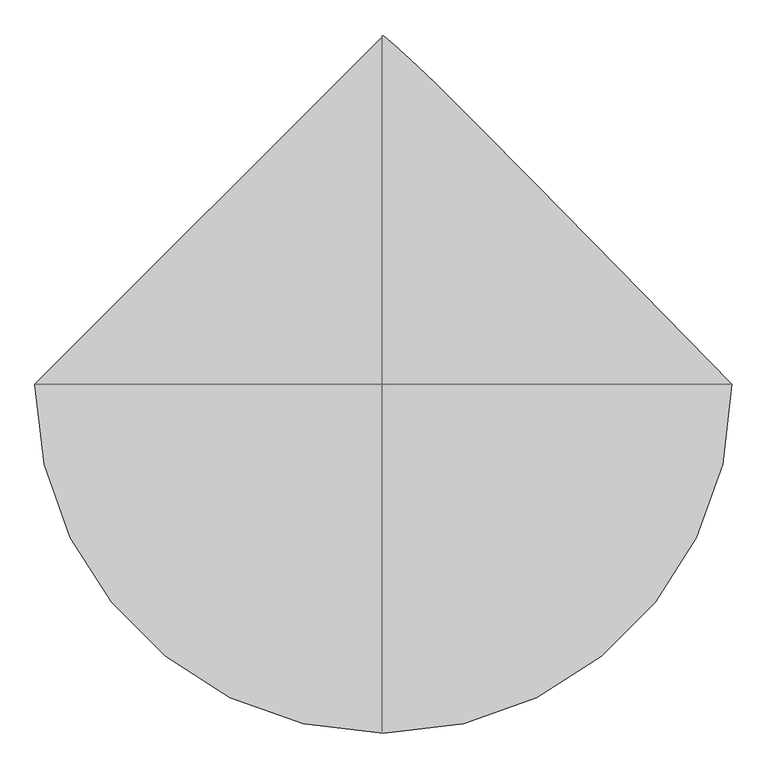
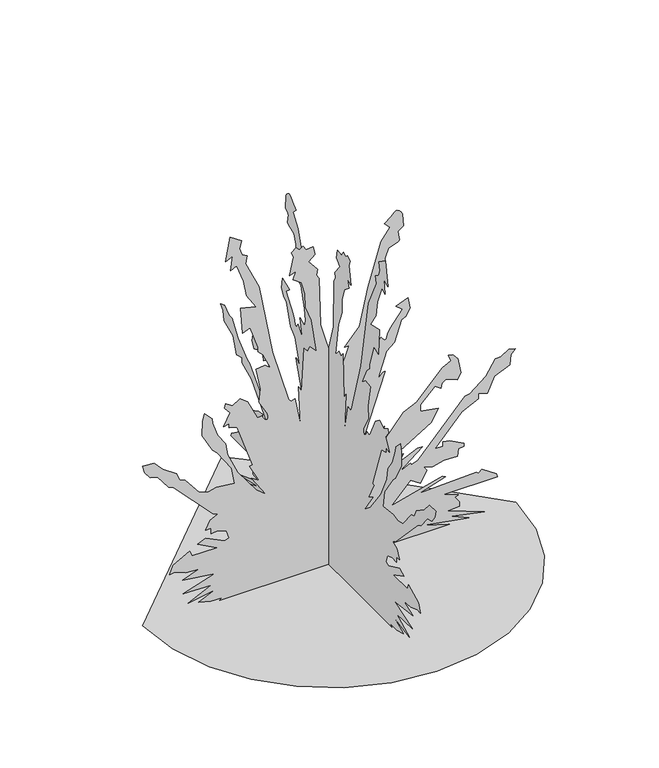
"""IFC4 building model written with IfcOpenShell, lengths in millimetres: proxy geometry, maiden grass 26738 : maiden grass 26738."""

import ifcopenshell
import ifcopenshell.guid

model = None  # the IFC model being written
_history = None  # IfcOwnerHistory: only IFC2X3 demands one
_inside = {}  # id of a spatial element -> (the spatial element, [elements in it])
_under = {}  # id of a project, library or spatial element -> (it, [spatial elements below it])
_declared = {}  # id of a project -> (the project, [libraries it declares])
_typed = {}  # id of a type object -> (the type object, [elements of that type])
_made_of = {}  # id of a material, layer set ... -> (it, [elements and type objects made of it])


def new_model(schema):
    """Start an empty IFC model of exactly this schema.

    Asked for "IFC4X3", IfcOpenShell would pick the latest addendum, in which some entities
    have other attributes; the version numbers below select the first issue.
    IFC2X3 requires an IfcOwnerHistory on every rooted entity: one is made here for all.
    """
    global model, _history
    if schema == "IFC4X3":
        model = ifcopenshell.file(schema_version=(4, 3, 0, 0))
    else:
        model = ifcopenshell.file(schema=schema)
    _inside.clear()
    _under.clear()
    _declared.clear()
    _typed.clear()
    _made_of.clear()
    _history = None
    if model.schema == "IFC2X3":
        org = make("IfcOrganization", Name="unknown")
        user = make(
            "IfcPersonAndOrganization",
            ThePerson=make("IfcPerson", FamilyName="unknown"),
            TheOrganization=org,
        )
        app = make(
            "IfcApplication",
            ApplicationDeveloper=org,
            Version="unknown",
            ApplicationFullName="unknown",
            ApplicationIdentifier="unknown",
        )
        _history = make(
            "IfcOwnerHistory",
            OwningUser=user,
            OwningApplication=app,
            ChangeAction="ADDED",
            CreationDate=0,
        )
    return model


def make(cls, **values):
    """One entity of the class cls with the attributes given. An attribute that is None is left unset."""
    return model.create_entity(
        cls, **{name: value for name, value in values.items() if value is not None}
    )


def rooted(cls, **values):
    """An entity with a GlobalId (a new one), such as an element, a storey or a relation."""
    return make(cls, GlobalId=ifcopenshell.guid.new(), OwnerHistory=_history, **values)


def si_unit(unit_type, name, prefix=None):
    """IfcSIUnit, for example si_unit("LENGTHUNIT", "METRE", prefix="MILLI")."""
    return make("IfcSIUnit", UnitType=unit_type, Prefix=prefix, Name=name)


def assignment(units):
    """IfcUnitAssignment: the units of a project."""
    return None if units is None else make("IfcUnitAssignment", Units=units)


def point(xyz):
    """IfcCartesianPoint."""
    return None if xyz is None else make("IfcCartesianPoint", Coordinates=xyz)


def direction(xyz):
    """IfcDirection."""
    return None if xyz is None else make("IfcDirection", DirectionRatios=xyz)


def frame(location, z_axis=None, x_axis=None):
    """IfcAxis2Placement3D, a coordinate frame: its origin and axes. An axis left out is left unset."""
    return make(
        "IfcAxis2Placement3D",
        Location=point(location),
        Axis=direction(z_axis),
        RefDirection=direction(x_axis),
    )


def origin():
    """The frame at (0, 0, 0) with its axes left unset."""
    return frame((0.0, 0.0, 0.0))


def place(relative_to, where):
    """IfcLocalPlacement: puts the frame where relative to a parent placement (None: the world)."""
    return make(
        "IfcLocalPlacement", PlacementRelTo=relative_to, RelativePlacement=where
    )


def context(
    kind, dimensions, precision=None, world=None, true_north=None, identifier=None
):
    """IfcGeometricRepresentationContext, for example the 3D "Model" context."""
    return make(
        "IfcGeometricRepresentationContext",
        ContextIdentifier=identifier,
        ContextType=kind,
        CoordinateSpaceDimension=dimensions,
        Precision=precision,
        WorldCoordinateSystem=world,
        TrueNorth=true_north,
    )


def project(units=None, contexts=None):
    """IfcProject with its units and contexts."""
    return rooted(
        "IfcProject",
        Name="project",
        RepresentationContexts=contexts,
        UnitsInContext=assignment(units),
    )


def spatial(cls, under=None, at=None, **own):
    """A site, building, storey or space (cls), placed at a placement, below another one or the project."""
    s = rooted(cls, ObjectPlacement=at, **own)
    if under is not None:
        _under.setdefault(under.id(), (under, []))[1].append(s)
    return s


def point_list(points):
    """IfcCartesianPointList2D or 3D."""
    cls = (
        "IfcCartesianPointList2D" if len(points[0]) == 2 else "IfcCartesianPointList3D"
    )
    return make(cls, CoordList=points)


def triangles(points, corners, closed=None, point_numbers=None):
    """IfcTriangulatedFaceSet: each triangle names its three corners, points numbered from 1."""
    return make(
        "IfcTriangulatedFaceSet",
        Coordinates=point_list(points),
        Closed=closed,
        CoordIndex=corners,
        PnIndex=point_numbers,
    )


def shape(context_of_items, identifier, shape_type, items):
    """IfcShapeRepresentation: the items that make up one representation, for example the "Body"."""
    return make(
        "IfcShapeRepresentation",
        ContextOfItems=context_of_items,
        RepresentationIdentifier=identifier,
        RepresentationType=shape_type,
        Items=items,
    )


def source(mapping_origin, context_of_items, identifier, shape_type, items):
    """IfcRepresentationMap: a shape defined once, which mapped items show again and again."""
    return make(
        "IfcRepresentationMap",
        MappingOrigin=mapping_origin,
        MappedRepresentation=shape(context_of_items, identifier, shape_type, items),
    )


def transform(
    local_origin,
    x_axis=None,
    y_axis=None,
    z_axis=None,
    scale=None,
    scale2=None,
    scale3=None,
    uniform=True,
):
    """IfcCartesianTransformationOperator3D, or its non-uniform kind. x_axis, y_axis, z_axis: its Axis1, 2, 3."""
    if uniform:
        return make(
            "IfcCartesianTransformationOperator3D",
            Axis1=direction(x_axis),
            Axis2=direction(y_axis),
            LocalOrigin=point(local_origin),
            Scale=scale,
            Axis3=direction(z_axis),
        )
    return make(
        "IfcCartesianTransformationOperator3DnonUniform",
        Axis1=direction(x_axis),
        Axis2=direction(y_axis),
        LocalOrigin=point(local_origin),
        Scale=scale,
        Axis3=direction(z_axis),
        Scale2=scale2,
        Scale3=scale3,
    )


def mapped(mapping_source, mapping_target):
    """IfcMappedItem: shows the shape of a source again, moved by a transform."""
    return make(
        "IfcMappedItem", MappingSource=mapping_source, MappingTarget=mapping_target
    )


def made_of(thing, what):
    """Note that an element or type object is made of a material, layer set ...; save() writes the relation."""
    if what is not None:
        _made_of.setdefault(what.id(), (what, []))[1].append(thing)
    return thing


def element(
    cls,
    number,
    at=None,
    inside=None,
    cuts=None,
    type_object=None,
    material=None,
    context=None,
    identifier="Body",
    shape_type=None,
    held_by="IfcProductDefinitionShape",
    body=None,
    shapes=None,
    **own,
):
    """One element of the class cls, such as IfcWall. Its Tag is "e" and its number.

    at: its placement. inside: the storey or other place that contains it. cuts: it is an
    opening in that element (IfcRelVoidsElement). A single representation is given by context,
    identifier, shape_type and body (its items); several are given by shapes. held_by: the class
    of the entity that holds the representations. save() writes the other relations.
    """
    e = rooted(cls, Tag="e%d" % number, ObjectPlacement=at, **own)
    if body is not None:
        shapes = [shape(context, identifier, shape_type, body)]
    if shapes is not None:
        e.Representation = make(held_by, Representations=shapes)
    if inside is not None:
        _inside.setdefault(inside.id(), (inside, []))[1].append(e)
    if cuts is not None:
        rooted(
            "IfcRelVoidsElement", RelatingBuildingElement=cuts, RelatedOpeningElement=e
        )
    if type_object is not None:
        _typed.setdefault(type_object.id(), (type_object, []))[1].append(e)
    return made_of(e, material)


def aggregate(whole, parts):
    """IfcRelAggregates: a whole, such as a stair, and the parts it consists of."""
    return rooted("IfcRelAggregates", RelatingObject=whole, RelatedObjects=parts)


def save(model, path):
    """Write the relations noted so far, then the file.

    IfcRelAggregates (storeys below a building ...), IfcRelContainedInSpatialStructure (elements
    in a storey), IfcRelDefinesByType, IfcRelAssociatesMaterial and IfcRelDeclares: one each for
    every whole, place, type object, material and project.
    """
    for whole, parts in _under.values():
        aggregate(whole, parts)
    for where, things in _inside.values():
        rooted(
            "IfcRelContainedInSpatialStructure",
            RelatedElements=things,
            RelatingStructure=where,
        )
    for kind, things in _typed.values():
        rooted("IfcRelDefinesByType", RelatedObjects=things, RelatingType=kind)
    for what, things in _made_of.values():
        rooted("IfcRelAssociatesMaterial", RelatedObjects=things, RelatingMaterial=what)
    for by, libraries in _declared.values():
        rooted("IfcRelDeclares", RelatingContext=by, RelatedDefinitions=libraries)
    model.write(path)


def entourage_51d93d44(model_context):
    return source(origin(), model_context, "Body", "Tessellation", [
        triangles([(-822.1126825, 0.0, 0.0001374), (-800.3786167, -188.373858, 0.0001374), (-738.480578, -361.3651156, 0.0001374), (-641.3745867, -514.0173532, 0.0001374), (-514.0174622, -641.374732, 0.0001374), (-361.365043, -738.4805054, 0.0001374), (-188.3737671, -800.378544, 0.0001374), (3.59e-05, -822.1126825, 0.0001374), (188.3739125, -800.3786167, 0.0001374), (361.3651883, -738.480578, 0.0001374), (514.0174622, -641.3745867, 0.0001374), (641.3748047, -514.0174622, 0.0001374), (738.4805054, -361.365043, 0.0001374), (800.378544, -188.373749, 0.0001374), (822.1126825, 7.19e-05, 0.0001374), (554.9441065, 274.0493697, 0.0001374), (356.8788342, 475.8195757, 0.0001374), (216.3996546, 617.3571573, 0.0001374), (121.9894107, 710.7087994, 0.0001374), (62.1308551, 767.9210049, 0.0001374), (25.3067606, 801.0401316, 0.0001374), (-0.0001078, 822.1126825, 0.0001374), (-486.0236403, 7.81e-05, 0.9155915), (-471.7920599, 7.76e-05, 9.8343198), (-523.9165309, 7.76e-05, 9.7573804), (-575.3383922, 7.67e-05, 24.6529329), (-504.1805263, 7.48e-05, 56.6647099), (-622.6670803, 7.61e-05, 35.566252), (-521.099806, 7.32e-05, 83.8197293), (-644.3685173, 7.29e-05, 88.7502968), (-506.307395, 7.03e-05, 133.1254316), (-645.8895727, 6.92e-05, 151.363835), (-575.3383922, 6.76e-05, 177.5005391), (-633.4720894, 6.73e-05, 182.811861), (-682.2468012, 6.62e-05, 200.8128698), (-703.5376528, 6.64e-05, 197.2227365), (-688.7453144, 6.41e-05, 236.667331), (-614.7840586, 6.17e-05, 276.1118528), (-604.9224512, 6.32e-05, 251.4590335), (-494.8790591, 6.34e-05, 248.9685605), (-580.2687962, 6.06e-05, 295.8341047), (-545.7534247, 5.97e-05, 310.6258072), (-461.9305979, 6.2e-05, 271.1812672), (-442.4802589, 6.16e-05, 277.8612192), (-452.1878423, 5.96e-05, 312.2414789), (-492.5862848, 5.87e-05, 327.4185685), (-520.7920123, 5.89e-05, 323.5701842), (-521.099806, 5.73e-05, 350.0703109), (-545.7534247, 5.73e-05, 350.0703109), (-526.0308277, 5.5e-05, 389.5148872), (-491.515202, 5.41e-05, 404.3065716), (-513.2632931, 5.35e-05, 414.7085166), (-685.7770363, 4.26e-05, 596.5231456), (-707.8857159, 4.2e-05, 606.6573017), (-757.7759846, 3.82e-05, 670.5571804), (-790.6316099, 3.78e-05, 677.9690826), (-814.6804327, 3.58e-05, 711.7275599), (-821.8761417, 3.38e-05, 744.5156021), (-771.5802292, 3.4e-05, 740.8769434), (-734.9066683, 3.66e-05, 698.0076851), (-673.9536301, 3.91e-05, 655.7654961), (-659.1609283, 4.12e-05, 621.2515417), (-636.2393623, 4.16e-05, 613.9256081), (-573.062332, 4.63e-05, 535.429927), (-531.2541281, 4.7e-05, 522.9600486), (-496.445933, 4.65e-05, 532.501254), (-417.5538008, 4.7e-05, 522.6401553), (-431.8794525, 4.26e-05, 597.7539207), (-494.1621334, 3.7e-05, 691.4321417), (-515.1618327, 3.58e-05, 710.6897598), (-560.6032451, 3.08e-05, 794.7286709), (-559.6332461, 2.68e-05, 861.8978268), (-550.6847371, 2.5e-05, 892.4327362), (-516.1688933, 2.71e-05, 857.9187092), (-514.4276842, 2.84e-05, 836.1371899), (-492.5786181, 3.21e-05, 773.1969183), (-456.9999032, 3.53e-05, 719.8628918), (-448.1073864, 3.85e-05, 666.0661755), (-403.8973306, 4.42e-05, 569.7717261), (-322.5198123, 5.08e-05, 459.5990905), (-279.4932235, 5.29e-05, 424.0288053), (-341.7963246, 4.73e-05, 518.5882951), (-309.0772825, 4.85e-05, 497.987336), (-351.6489936, 4.37e-05, 579.3482491), (-338.6617049, 4.35e-05, 581.8069654), (-407.6923751, 3.18e-05, 779.0296291), (-442.2077102, 3.12e-05, 788.8907278), (-442.2077102, 3e-05, 808.6129978), (-466.8613289, 3.03e-05, 803.6824848), (-437.2769065, 2.71e-05, 857.9187092), (-461.9305979, 2.53e-05, 887.5020779), (-456.9999032, 2.41e-05, 907.2244205), (-427.4157715, 2.53e-05, 887.5020779), (-392.9001457, 2.41e-05, 907.2244205), (-361.3909862, 2.55e-05, 883.444622), (-319.5289701, 3.13e-05, 794.863619), (-316.5251201, 3.15e-05, 792.847681), (-312.9193082, 3.15e-05, 792.290593), (-308.9018935, 3.15e-05, 792.6843916), (-304.6633259, 3.13e-05, 793.5212591), (-300.3935829, 3.11e-05, 794.293523), (-296.2831507, 3.08e-05, 794.4932928), (-293.8821344, 3.1e-05, 789.7024515), (-291.6524922, 3.11e-05, 784.6016001), (-289.2939152, 3.13e-05, 779.6455799), (-286.5060222, 3.14e-05, 775.2894505), (-282.9887042, 3.16e-05, 771.9882711), (-278.4414163, 3.19e-05, 770.1969561), (-272.5639226, 3.23e-05, 770.3705647), (-270.4821274, 3.19e-05, 776.4802935), (-269.746798, 3.16e-05, 782.5422054), (-271.4178988, 3.09e-05, 794.5538269), (-309.0772825, 2.68e-05, 862.8492222), (-304.1468967, 2.32e-05, 922.0159595), (-323.8695119, 1.74e-05, 1020.6273823), (-284.423464, 1.71e-05, 1025.5578953), (-259.7697544, 1.82e-05, 1005.8357706), (-292.5143764, 1.4e-05, 1076.7667608), (-314.0080499, 1.27e-05, 1099.5164623), (-315.0547156, 1.15e-05, 1119.0795851), (-348.5233486, 5.3e-06, 1222.7807407), (-383.038502, 6.2e-06, 1207.9888384), (-391.1781941, -1e-06, 1327.8346481), (-323.8695119, 0.0, 1311.5309921), (-365.2547038, -3.9e-06, 1377.9884182), (-377.5616561, -8.2e-06, 1449.0455635), (-409.7759325, -1.31e-05, 1532.0531422), (-435.1933854, -1.24e-05, 1519.3450516), (-427.4157715, -1.61e-05, 1582.7118233), (-456.9999032, -1.53e-05, 1567.9204296), (-438.6445556, -2.17e-05, 1676.3998547), (-387.9694147, -1.97e-05, 1641.8788513), (-396.0815286, -1.75e-05, 1605.9381672), (-384.2218237, -1.56e-05, 1574.3406773), (-363.3155416, -1.5e-05, 1562.9896259), (-368.246309, -1.29e-05, 1528.4758896), (-309.0772825, -5.3e-06, 1400.2812435), (-250.6196225, 1.42e-05, 1073.5192846), (-180.2010283, 2.87e-05, 830.6251717), (-169.6161911, 2.95e-05, 817.4087545), (-151.2930636, 2.91e-05, 823.4046822), (-126.6192335, 3.68e-05, 694.4196774), (-136.5008433, 2.62e-05, 872.7103935), (-121.7086412, 2.76e-05, 848.0576105), (-111.8470156, 1.59e-05, 1045.2803106), (-97.0548044, 1.71e-05, 1025.5578953), (-84.6295182, 1.62e-05, 1040.6290684), (-57.6092516, 1.79e-05, 1010.7662109), (-79.5582798, 8.8e-06, 1163.7574539), (-104.4511553, 4.7e-06, 1232.6419121), (-107.5404289, 9e-07, 1296.0368797), (-123.4986664, -2.4e-06, 1352.177639), (-161.1545347, -4.1e-06, 1380.5586102), (-146.3623326, -6.2e-06, 1415.0727825), (-175.9469094, -5.6e-06, 1405.2116112), (-158.7234512, -1.03e-05, 1484.8167812), (-166.0854474, -1.17e-05, 1508.7534016), (-146.3623326, -1.26e-05, 1523.5452312), (-131.5704484, -1.17e-05, 1508.7534016), (-116.6065998, -1.25e-05, 1521.4754448), (-101.9855355, -1.11e-05, 1498.8923756), (-72.4009586, -1.14e-05, 1503.8230339), (-62.5394784, -9.1e-06, 1464.3783485), (-92.1240644, -7.6e-06, 1439.7256382), (-52.6780073, -4.7e-06, 1390.4200722), (-57.6092516, -3.2e-06, 1365.7670712), (-44.9584885, -2.1e-06, 1346.546006), (-40.1288097, 1.1e-05, 1128.143712), (16.3521246, 2.24e-05, 936.8077166), (25.6302442, 2.16e-05, 950.3199005), (46.3616142, 2.59e-05, 877.5758669), (85.383115, 1.94e-05, 986.1135006), (65.6596505, 1.94e-05, 986.1135006), (132.852038, 1.49e-05, 1062.0039265), (169.7376772, 4.9e-06, 1229.8971668), (228.245861, -6.6e-06, 1421.9566647), (267.8211162, -9.7e-06, 1474.2395199), (243.1672431, -1.11e-05, 1498.8923756), (272.0833378, -1.25e-05, 1521.3225471), (286.4673436, -1.31e-05, 1537.556876), (293.7374485, -1.35e-05, 1542.3155972), (297.4055931, -1.38e-05, 1543.2675739), (308.1376596, -1.27e-05, 1537.579549), (315.8437663, -1.16e-05, 1529.0826839), (321.0283699, -1.07e-05, 1518.2452641), (326.6370392, -7.7e-06, 1460.8509476), (306.7311321, -7.7e-06, 1447.4507481), (304.3311514, -7.7e-06, 1444.519241), (302.7936726, -7.7e-06, 1441.4505329), (309.1859605, -6.2e-06, 1402.4600349), (307.1584316, -5.9e-06, 1398.4450184), (302.9130694, -5.6e-06, 1394.7411747), (261.356885, -4e-06, 1379.0709103), (246.0123274, -1.6e-06, 1337.9506004), (244.0019305, 9e-07, 1296.3149151), (228.3094291, 3.3e-06, 1256.0202816), (220.8882069, 7.9e-06, 1179.9705631), (207.4437332, 6.8e-06, 1171.8723656), (179.3911032, 1.38e-05, 1079.9680189), (173.3980279, 1.7e-05, 1026.8490955), (180.4457445, 1.86e-05, 999.5491631), (213.582312, 1.77e-05, 1015.6967239), (193.859715, 2.26e-05, 931.8771309), (228.3750501, 2e-05, 976.2522566), (242.287573, 2.11e-05, 957.5074705), (251.845438, 2.09e-05, 961.1874784), (256.8526723, 1.97e-05, 980.8979033), (266.7142615, 1.85e-05, 1002.0413801), (322.059448, 1.41e-05, 1074.863534), (293.6769507, 1.28e-05, 1097.3908653), (346.713212, 1.15e-05, 1119.2386597), (354.6484835, 1.44e-05, 1069.6418324), (338.174271, 1.65e-05, 1035.8738354), (317.1287169, 1.71e-05, 1025.5578953), (287.5436224, 2.26e-05, 931.8771309), (252.1265254, 2.44e-05, 903.2333851), (213.582312, 3.12e-05, 788.8907278), (236.8349806, 3.03e-05, 809.7009401), (240.9621815, 3e-05, 811.6948591), (244.803971, 2.97e-05, 812.5061468), (244.8585279, 3e-05, 809.5433916), (134.690634, 4.91e-05, 488.1261283), (242.8606121, 4.5e-05, 557.2269977), (237.4122891, 4.6e-05, 540.8212403), (140.9250282, 5.13e-05, 450.6353934), (129.759903, 5.23e-05, 433.8900129), (164.2748021, 5.06e-05, 463.4733816), (174.1367001, 5.06e-05, 463.4733816), (159.0154937, 5.29e-05, 425.0493098), (238.8042827, 4.92e-05, 486.724506), (326.990179, 4.29e-05, 591.668064), (382.9130736, 4.13e-05, 618.7366516), (499.039125, 3.41e-05, 739.7414022), (534.9049227, 3.29e-05, 759.6449112), (524.2203278, 3.12e-05, 788.8907278), (544.510332, 3.15e-05, 783.3986212), (566.5761726, 3.31e-05, 756.7437075), (580.5672881, 3.72e-05, 688.0601091), (563.6663939, 3.88e-05, 660.6960091), (514.5438108, 3.76e-05, 681.3525244), (496.7209162, 3.83e-05, 668.9436161), (492.0994686, 3.96e-05, 646.9967726), (465.0513376, 3.85e-05, 665.6265947), (400.9515075, 4.23e-05, 601.5291627), (400.9515075, 4.41e-05, 571.9458303), (479.8436033, 4.5e-05, 557.154146), (450.2590719, 4.82e-05, 502.9179216), (287.5436224, 5.41e-05, 404.3065716), (325.8399585, 5.44e-05, 399.649116), (302.3363241, 5.64e-05, 364.8620679), (387.4521134, 5.41e-05, 404.7523293), (411.1211992, 5.41e-05, 403.6902938), (307.2671459, 5.91e-05, 320.4869785), (356.5747104, 5.76e-05, 345.1397979), (361.5048964, 5.82e-05, 335.2785539), (389.4130039, 5.74e-05, 348.2994524), (598.1816563, 4.41e-05, 571.9458303), (618.663909, 4.38e-05, 576.9850576), (688.6817282, 4.05e-05, 633.1896212), (731.3115389, 3.65e-05, 700.1405491), (755.9652666, 3.65e-05, 700.1405491), (790.4811104, 3.5e-05, 724.7934048), (820.0657145, 3.56e-05, 714.9323061), (800.3426451, 3.68e-05, 695.2100361), (795.4119141, 3.94e-05, 650.8349104), (726.3813166, 4.12e-05, 621.2515417), (696.7968578, 4.53e-05, 552.2235603), (657.3502831, 4.47e-05, 562.084659), (657.4310921, 4.61e-05, 538.9833801), (583.1111009, 4.8e-05, 506.1758986), (465.0513376, 5.59e-05, 374.7231666), (499.5666, 5.59e-05, 374.7231666), (499.5666, 5.47e-05, 394.4454366), (528.894134, 5.5e-05, 389.8867032), (593.2509616, 5.7e-05, 355.0009329), (593.2509616, 5.79e-05, 340.2092485), (568.4129791, 5.81e-05, 337.6585321), (563.6663939, 6e-05, 305.6952579), (504.8713271, 5.99e-05, 306.2484581), (453.6921109, 6.06e-05, 295.5878443), (415.7437732, 6e-05, 305.6952579), (430.5360752, 6.11e-05, 285.9729515), (400.9515075, 6.41e-05, 236.667331), (356.5747104, 6.23e-05, 266.2507178), (272.7518472, 6.76e-05, 177.5005391), (498.0560818, 6.42e-05, 234.1173413), (512.2016573, 6.46e-05, 227.2681409), (396.0207401, 6.67e-05, 192.2922235), (647.8657602, 6.62e-05, 201.1622852), (657.3502831, 6.67e-05, 192.2922235), (672.1430574, 6.59e-05, 207.083926), (736.2428513, 6.85e-05, 162.7088003), (741.1735823, 6.94e-05, 147.9171159), (499.5666, 6.94e-05, 147.9171159), (568.5971612, 7.08e-05, 123.2642602), (552.2703235, 7.12e-05, 117.9041314), (573.5278922, 7.29e-05, 88.7502968), (573.5278922, 7.41e-05, 69.0280223), (521.428892, 7.43e-05, 64.9850141), (682.0040108, 7.79e-05, 4.9306691), (539.0127025, 7.61e-05, 34.5140656), (617.9047256, 7.82e-05, 0.0001036), (415.7437732, 7.61e-05, 34.5140656), (529.1511314, 7.82e-05, 0.0001036), (-3.5682026, -482.4553988, 0.9154881), (-3.5682026, -468.2238184, 9.8342176), (-3.5682026, -520.3482894, 9.7572771), (-3.5682026, -571.770187, 24.652833), (-3.5682026, -500.6122484, 56.6646145), (-3.5682026, -619.0989115, 35.5661476), (-3.5682026, -517.5314919, 83.8196294), (-3.5682026, -640.8002758, 88.750206), (-3.5682026, -502.7391898, 133.1253407), (-3.5682026, -642.3213312, 151.3637533), (-3.5682026, -571.770187, 177.5004483), (-3.5682026, -629.9037752, 182.8117702), (-3.5682026, -678.6785597, 200.8127971), (-3.5682026, -699.9694839, 197.2226638), (-3.5682026, -685.1770729, 236.6672583), (-3.5682026, -611.2158897, 276.1117802), (-3.5682026, -601.3542097, 251.4589427), (-3.5682026, -491.310854, 248.9684878), (-3.5682026, -576.7005547, 295.8340138), (-3.5682026, -542.1852559, 310.6257345), (-3.5682026, -458.3623564, 271.1812308), (-3.5682026, -438.9119811, 277.8611647), (-3.5682026, -448.6196008, 312.2414426), (-3.5682026, -489.0179707, 327.4185322), (-3.5682026, -517.2238071, 323.5701479), (-3.5682026, -517.5314919, 350.0702745), (-3.5682026, -542.1852559, 350.0702745), (-3.5682026, -522.4626225, 389.5148509), (-3.5682026, -487.9469604, 404.3065352), (-3.5682026, -509.6950516, 414.7084803), (-3.5682026, -682.2087948, 596.5231456), (-3.5682026, -704.3174744, 606.6573017), (-3.5682026, -754.2077431, 670.5571804), (-3.5682026, -787.0633684, 677.9690826), (-3.5682026, -811.1121912, 711.7275599), (-3.5682026, -818.3079729, 744.5156021), (-3.5682026, -768.0119877, 740.8769434), (-3.5682026, -731.3384995, 698.0076851), (-3.5682026, -670.3853886, 655.7654961), (-3.5682026, -655.5926868, 621.251469), (-3.5682026, -632.6711208, 613.9256081), (-3.5682026, -569.4940905, 535.4298543), (-3.5682026, -527.6859229, 522.9599759), (-3.5682026, -492.8777278, 532.501254), (-3.5682026, -413.9855593, 522.6401553), (-3.5682026, -428.311211, 597.7538844), (-3.5682026, -490.5938556, 691.4321417), (-3.5682026, -511.5936275, 710.6897598), (-3.5682026, -557.0350036, 794.7286709), (-3.5682026, -556.0649683, 861.8978268), (-3.5682026, -547.1164956, 892.4327362), (-3.5682026, -512.6006518, 857.9187092), (-3.5682026, -510.85937, 836.1371899), (-3.5682026, -489.0103766, 773.1969183), (-3.5682026, -453.4316254, 719.8628918), (-3.5682026, -444.5391449, 666.0661028), (-3.5682026, -400.3290891, 569.7716535), (-3.5682026, -318.9515708, 459.5990541), (-3.5682026, -275.9250001, 424.0287689), (-3.5682026, -338.2281195, 518.5882224), (-3.5682026, -305.5090774, 497.9872996), (-3.5682026, -348.0807884, 579.3482491), (-3.5682026, -335.0934634, 581.8069654), (-3.5682026, -404.1241336, 779.0296291), (-3.5682026, -438.6394687, 788.8907278), (-3.5682026, -438.6394687, 808.6129978), (-3.5682026, -463.2930874, 803.6824848), (-3.5682026, -433.7087377, 857.9187092), (-3.5682026, -458.3623564, 887.5020779), (-3.5682026, -453.4316254, 907.2244205), (-3.5682026, -423.84753, 887.5020779), (-3.5682026, -389.3319042, 907.2244205), (-3.5682026, -357.8227083, 883.444622), (-3.5682026, -315.9607286, 794.863619), (-3.5682026, -312.9568422, 792.847681), (-3.5682026, -309.351103, 792.290593), (-3.5682026, -305.3336884, 792.6843916), (-3.5682026, -301.0950844, 793.5212591), (-3.5682026, -296.8253414, 794.293523), (-3.5682026, -292.7149092, 794.4932928), (-3.5682026, -290.3138929, 789.7024515), (-3.568202, -288.0842507, 784.6016001), (-3.568202, -285.7257101, 779.6455799), (-3.568202, -282.9377988, 775.2894505), (-3.568202, -279.4204808, 771.9882711), (-3.568202, -274.873193, 770.1969561), (-3.5682026, -268.9956993, 770.3705647), (-3.5682026, -266.9138678, 776.4802935), (-3.5682026, -266.1785747, 782.5422054), (-3.5682026, -267.8496573, 794.5538269), (-3.5682026, -305.5090774, 862.8492222), (-3.5682026, -300.5786552, 922.0161776), (-3.5682026, -320.3012704, 1020.6273823), (-3.5682026, -280.8552043, 1025.5579679), (-3.5682026, -256.2015129, 1005.8357706), (-3.5682026, -288.946153, 1076.7667608), (-3.5682026, -310.4398084, 1099.5164623), (-3.5682026, -311.4864741, 1119.0795851), (-3.5682026, -344.9551071, 1222.7807407), (-3.5682026, -379.4702605, 1207.9888384), (-3.5682026, -387.6099526, 1327.8347935), (-3.5682026, -320.3012704, 1311.5309921), (-3.5682026, -361.6864986, 1377.9885635), (-3.5682026, -373.9934146, 1449.0455635), (-3.5682026, -406.2076547, 1532.0531422), (-3.5682026, -431.6251802, 1519.3451969), (-3.5682026, -423.84753, 1582.712114), (-3.5682026, -453.4316254, 1567.9204296), (-3.5682026, -435.0763867, 1676.4), (-3.5682026, -384.4011732, 1641.8788513), (-3.5682026, -392.5132507, 1605.9383125), (-3.5682026, -380.6535822, 1574.3408226), (-3.5682026, -359.7473365, 1562.9896259), (-3.5682026, -364.6781038, 1528.4760349), (-3.5682026, -305.5090774, 1400.2812435), (-3.5682026, -247.0513992, 1073.5192846), (-3.5682026, -176.632805, 830.6251717), (-3.5682026, -166.0479678, 817.4087545), (-3.5682026, -147.7248221, 823.4047548), (-3.5682026, -123.0510011, 694.4196774), (-3.5682026, -132.93262, 872.7103935), (-3.5682026, -118.1404088, 848.0576105), (-3.5682026, -108.2787832, 1045.2803833), (-3.5682026, -93.486572, 1025.5579679), (-3.5682026, -81.0612858, 1040.6290684), (-3.5682026, -54.0410146, 1010.7662109), (-3.5682026, -75.9900428, 1163.7574539), (-3.5682026, -100.8829229, 1232.6419121), (-3.5682026, -103.9721874, 1296.0368797), (-3.5682026, -119.9304249, 1352.177639), (-3.5682026, -157.5863113, 1380.5587555), (-3.5682026, -142.7940911, 1415.0729279), (-3.5682026, -172.3786679, 1405.2117565), (-3.5682026, -155.1552097, 1484.8169266), (-3.5682026, -162.517224, 1508.7536922), (-3.5682026, -142.7940911, 1523.5453766), (-3.5682026, -128.002225, 1508.7536922), (-3.5682026, -113.0383673, 1521.4754448), (-3.5682026, -98.417303, 1498.8925209), (-3.5682026, -68.8327217, 1503.8230339), (-3.5682026, -58.9712415, 1464.3784939), (-3.5682026, -88.5558228, 1439.7256382), (-3.5682026, -49.1097749, 1390.4200722), (-3.5682026, -54.0410146, 1365.7670712), (-3.5682026, -41.3902516, 1346.5461514), (-3.5682026, -36.560575, 1128.143712), (-3.5682026, 19.9203638, 936.8078619), (-3.5682026, 29.1984812, 950.3199005), (-3.5682026, 49.9298511, 877.5758669), (-3.5682026, 88.9513474, 986.1135006), (-3.5682026, 69.2278874, 986.1135006), (-3.5682026, 136.4202886, 1062.0039991), (-3.5682026, 173.3059187, 1229.8973122), (-3.5682026, 231.8141025, 1421.95681), (-3.5682026, 271.3893577, 1474.2395199), (-3.5682026, 246.7355028, 1498.8925209), (-3.5682026, 275.6515793, 1521.3226925), (-3.5682026, 290.0355851, 1537.5570213), (-3.5682026, 297.30569, 1542.3158878), (-3.5682026, 300.9738527, 1543.2675739), (-3.5682032, 311.7059011, 1537.5796944), (-3.5682035, 319.4120078, 1529.0828293), (-3.568204, 324.5966477, 1518.2452641), (-3.5682035, 330.2052807, 1460.8509476), (-3.5682026, 310.2993736, 1447.4507481), (-3.5682026, 307.8994111, 1444.5193863), (-3.5682026, 306.3618959, 1441.4505329), (-3.5682015, 312.754202, 1402.4600349), (-3.5682015, 310.7266368, 1398.4451637), (-3.5682015, 306.4812927, 1394.74132), (-3.5682026, 264.9251265, 1379.0710556), (-3.5682026, 249.5805508, 1337.9507458), (-3.5682026, 247.5701539, 1296.3149151), (-3.5682026, 231.8776706, 1256.0204269), (-3.5682026, 224.4564302, 1179.9705631), (-3.5682012, 211.0119747, 1171.8725836), (-3.5682026, 182.9593447, 1079.9680189), (-3.5682026, 176.9662694, 1026.8490955), (-3.5682026, 184.0139678, 999.5491631), (-3.5682026, 217.1505535, 1015.6968693), (-3.5682026, 197.4279383, 931.8772036), (-3.5682026, 231.9432552, 976.2522566), (-3.5682026, 245.8557963, 957.5075432), (-3.5682026, 255.4136795, 961.1876965), (-3.5682026, 260.4209138, 980.8979033), (-3.5682026, 270.2824848, 1002.0413801), (-3.5682026, 325.6276895, 1074.863534), (-3.5682026, 297.2451922, 1097.3908653), (-3.5682026, 350.2814172, 1119.2386597), (-3.5682026, 358.216725, 1069.6418324), (-3.5682026, 341.7425125, 1035.8738354), (-3.5682026, 320.6969584, 1025.5579679), (-3.5682026, 291.1118639, 931.8772036), (-3.5682026, 255.694767, 903.2333851), (-3.5682026, 217.1505535, 788.8907278), (-3.5682026, 240.4032221, 809.7009401), (-3.5682026, 244.5303866, 811.6948591), (-3.5682026, 248.3722125, 812.5061468), (-3.5682026, 248.4268058, 809.5433916), (-3.5682026, 138.2588664, 488.1261283), (-3.5682026, 246.4288173, 557.2269613), (-3.5682026, 240.9805125, 540.8212403), (-3.5682026, 144.4932697, 450.6353208), (-3.5682026, 133.3281354, 433.8899766), (-3.5682026, 167.8430436, 463.4733089), (-3.5682026, 177.7049234, 463.4733089), (-3.5682026, 162.5837171, 425.0492735), (-3.5682026, 242.3725242, 486.724397), (-3.5682026, 330.5584205, 591.668064), (-3.5682026, 386.4813151, 618.7366516), (-3.5682026, 502.6072938, 739.7414022), (-3.5682026, 538.4731278, 759.6449112), (-3.5682026, 527.7886419, 788.8907278), (-3.5682026, 548.0786098, 783.3986212), (-3.5682026, 570.1443778, 756.7437075), (-3.5682026, 584.1354933, 688.0601091), (-3.5682026, 567.2346717, 660.6960091), (-3.5682026, 518.112016, 681.3525244), (-3.5682026, 500.2891577, 668.9436161), (-3.5682026, 495.6677828, 646.9966999), (-3.5682026, 468.6195791, 665.6265947), (-3.5682026, 404.519749, 601.5291264), (-3.5682026, 404.519749, 571.9457577), (-3.5682026, 483.4118448, 557.1540733), (-3.5682026, 453.8273134, 502.917849), (-3.5682026, 291.1118639, 404.3065352), (-3.5682026, 329.4082363, 399.6490434), (-3.5682026, 305.9045837, 364.8620316), (-3.5682026, 391.0203549, 404.7522566), (-3.5682026, 414.6894407, 403.6902211), (-3.5682026, 310.8353874, 320.4869059), (-3.5682026, 360.1429519, 345.1397615), (-3.5682026, 365.0731379, 335.2785539), (-3.5682026, 392.9812454, 348.2994161), (-3.5682026, 601.7499341, 571.9457577), (-3.5682026, 622.2321505, 576.9850576), (-3.5682026, 692.2499697, 633.1895485), (-3.5682026, 734.8797804, 700.1405491), (-3.5682026, 759.5335808, 700.1405491), (-3.5682026, 794.0494246, 724.7934048), (-3.5682026, 823.6338106, 714.9323061), (-3.5682026, 803.9108866, 695.2100361), (-3.5682026, 798.9800829, 650.8349104), (-3.5682026, 729.9495581, 621.251469), (-3.5682026, 700.3650267, 552.223524), (-3.5682026, 660.9185246, 562.084659), (-3.5682026, 660.9993336, 538.9833801), (-3.5682026, 586.679306, 506.175826), (-3.5682026, 468.6195791, 374.7231302), (-3.5682026, 503.1348415, 374.7231302), (-3.5682026, 503.1348415, 394.4453639), (-3.5682026, 532.4624119, 389.8866669), (-3.5682026, 596.8191668, 355.0008602), (-3.5682026, 596.8191668, 340.2091759), (-3.5682026, 571.981257, 337.6584958), (-3.5682026, 567.2346717, 305.6951852), (-3.5682026, 508.4395686, 306.2483854), (-3.5682026, 457.2603161, 295.5877898), (-3.5682026, 419.3120147, 305.6951852), (-3.5682026, 434.1043167, 285.9729152), (-3.5682026, 404.519749, 236.6672583), (-3.5682026, 360.1429519, 266.2506452), (-3.5682026, 276.3200705, 177.5004483), (-3.5682026, 501.6243959, 234.1172686), (-3.5682026, 515.7698625, 227.2680864), (-3.5682026, 399.5889816, 192.2921508), (-3.5682026, 651.4340017, 201.1622126), (-3.5682026, 660.9185246, 192.2921508), (-3.5682026, 675.7112989, 207.0838533), (-3.5682026, 739.8110928, 162.7087094), (-3.5682026, 744.7418238, 147.9170433), (-3.5682026, 503.1348415, 147.9170433), (-3.5682026, 572.1653664, 123.2641785), (-3.5682026, 555.8386013, 117.9040406), (-3.5682026, 577.0961337, 88.750206), (-3.5682026, 577.0961337, 69.027936), (-3.5682026, 524.9970972, 64.9849233), (-3.5682026, 685.5723249, 4.9305664), (-3.5682026, 542.5808713, 34.5139657), (-3.5682026, 621.4728945, 0.0), (-3.5682026, 419.3120147, 34.5139657), (-3.5682026, 532.7193003, 0.0)], [[21, 22, 1], [20, 21, 1], [19, 20, 1], [18, 19, 1], [17, 18, 1], [17, 1, 2], [17, 2, 3], [17, 3, 4], [16, 17, 4], [16, 4, 5], [16, 5, 6], [16, 6, 7], [16, 7, 8], [16, 8, 9], [16, 9, 10], [16, 10, 11], [16, 11, 12], [15, 16, 12], [14, 15, 12], [13, 14, 12], [299, 300, 301], [301, 302, 303], [27, 28, 29], [303, 304, 23], [29, 30, 31], [81, 82, 83], [31, 32, 33], [142, 143, 144], [303, 23, 24], [294, 295, 296], [222, 223, 224], [144, 145, 146], [25, 26, 27], [251, 252, 253], [250, 251, 253], [286, 287, 288], [285, 286, 288], [222, 224, 225], [172, 173, 174], [88, 89, 90], [169, 170, 171], [201, 202, 203], [40, 41, 42], [40, 42, 43], [129, 130, 131], [129, 131, 132], [129, 132, 133], [234, 235, 236], [154, 155, 156], [127, 128, 129], [35, 36, 37], [299, 301, 303], [209, 210, 211], [209, 211, 212], [72, 73, 74], [234, 236, 237], [248, 249, 250], [262, 263, 264], [48, 49, 50], [24, 25, 27], [241, 242, 243], [292, 293, 294], [227, 228, 229], [226, 227, 229], [91, 92, 93], [90, 91, 93], [121, 122, 123], [121, 123, 124], [245, 246, 247], [261, 262, 264], [209, 212, 213], [208, 209, 213], [208, 213, 214], [208, 214, 215], [207, 208, 215], [206, 207, 215], [83, 84, 85], [57, 58, 59], [129, 133, 134], [127, 129, 134], [203, 204, 205], [206, 215, 216], [205, 206, 216], [203, 205, 216], [219, 220, 221], [272, 273, 274], [146, 147, 148], [144, 146, 148], [159, 160, 161], [140, 141, 142], [177, 178, 179], [46, 47, 48], [37, 38, 39], [71, 72, 74], [71, 74, 75], [71, 75, 76], [70, 71, 76], [70, 76, 77], [69, 70, 77], [69, 77, 78], [68, 69, 78], [68, 78, 79], [67, 68, 79], [67, 79, 80], [245, 247, 248], [114, 115, 116], [114, 116, 117], [282, 283, 284], [281, 282, 284], [56, 57, 59], [56, 59, 60], [55, 56, 60], [35, 37, 39], [34, 35, 39], [33, 34, 39], [33, 39, 40], [31, 33, 40], [253, 254, 255], [261, 264, 265], [261, 265, 266], [260, 261, 266], [259, 260, 266], [259, 266, 267], [258, 259, 267], [258, 267, 268], [127, 134, 135], [127, 135, 136], [126, 127, 136], [126, 136, 137], [125, 126, 137], [124, 125, 137], [124, 137, 138], [121, 124, 138], [120, 121, 138], [119, 120, 138], [118, 119, 138], [117, 118, 138], [117, 138, 139], [114, 117, 139], [113, 114, 139], [112, 113, 139], [297, 298, 299], [296, 297, 299], [294, 296, 299], [294, 299, 303], [161, 162, 163], [161, 163, 164], [55, 60, 61], [54, 55, 61], [54, 61, 62], [53, 54, 62], [52, 53, 62], [52, 62, 63], [52, 63, 64], [52, 64, 65], [275, 276, 277], [274, 275, 277], [52, 65, 66], [52, 66, 67], [51, 52, 67], [51, 67, 80], [203, 216, 217], [277, 278, 279], [274, 277, 279], [272, 274, 279], [271, 272, 279], [271, 279, 280], [271, 280, 281], [157, 158, 159], [156, 157, 159], [238, 239, 240], [237, 238, 240], [234, 237, 240], [233, 234, 240], [290, 291, 292], [290, 292, 294], [289, 290, 294], [288, 289, 294], [288, 294, 303], [288, 303, 24], [285, 288, 24], [112, 139, 140], [112, 140, 142], [111, 112, 142], [110, 111, 142], [109, 110, 142], [152, 153, 154], [218, 219, 221], [217, 218, 221], [217, 221, 222], [86, 87, 88], [48, 50, 51], [46, 48, 51], [46, 51, 80], [45, 46, 80], [45, 80, 81], [44, 45, 81], [233, 240, 241], [233, 241, 243], [233, 243, 244], [232, 233, 244], [231, 232, 244], [231, 244, 245], [231, 245, 248], [230, 231, 248], [229, 230, 248], [258, 268, 269], [258, 269, 270], [257, 258, 270], [256, 257, 270], [256, 270, 271], [256, 271, 281], [256, 281, 284], [255, 256, 284], [253, 255, 284], [253, 284, 285], [285, 24, 27], [253, 285, 27], [250, 253, 27], [248, 250, 27], [229, 248, 27], [226, 229, 27], [226, 27, 29], [226, 29, 31], [226, 31, 40], [226, 40, 43], [226, 43, 44], [226, 44, 81], [226, 81, 83], [93, 94, 95], [90, 93, 95], [88, 90, 95], [86, 88, 95], [85, 86, 95], [85, 95, 96], [85, 96, 97], [85, 97, 98], [85, 98, 99], [85, 99, 100], [85, 100, 101], [85, 101, 102], [85, 102, 103], [85, 103, 104], [85, 104, 105], [85, 105, 106], [85, 106, 107], [85, 107, 108], [85, 108, 109], [85, 109, 142], [83, 85, 142], [226, 83, 142], [225, 226, 142], [222, 225, 142], [217, 222, 142], [217, 142, 144], [159, 161, 164], [156, 159, 164], [154, 156, 164], [152, 154, 164], [152, 164, 165], [152, 165, 166], [151, 152, 166], [151, 166, 167], [150, 151, 167], [150, 167, 168], [149, 150, 168], [148, 149, 168], [148, 168, 169], [144, 148, 169], [144, 169, 171], [217, 144, 171], [203, 217, 171], [203, 171, 172], [201, 203, 172], [201, 172, 174], [200, 201, 174], [199, 200, 174], [199, 174, 175], [198, 199, 175], [197, 198, 175], [196, 197, 175], [196, 175, 176], [195, 196, 176], [194, 195, 176], [193, 194, 176], [193, 176, 177], [192, 193, 177], [191, 192, 177], [190, 191, 177], [189, 190, 177], [188, 189, 177], [187, 188, 177], [187, 177, 179], [186, 187, 179], [185, 186, 179], [184, 185, 179], [183, 184, 179], [182, 183, 179], [182, 179, 180], [182, 180, 181], [581, 582, 583], [583, 584, 585], [309, 310, 311], [585, 586, 305], [311, 312, 313], [363, 364, 365], [313, 314, 315], [424, 425, 426], [585, 305, 306], [576, 577, 578], [504, 505, 506], [426, 427, 428], [307, 308, 309], [533, 534, 535], [532, 533, 535], [568, 569, 570], [567, 568, 570], [504, 506, 507], [454, 455, 456], [370, 371, 372], [451, 452, 453], [483, 484, 485], [322, 323, 324], [322, 324, 325], [411, 412, 413], [411, 413, 414], [411, 414, 415], [516, 517, 518], [436, 437, 438], [409, 410, 411], [317, 318, 319], [581, 583, 585], [491, 492, 493], [491, 493, 494], [354, 355, 356], [516, 518, 519], [530, 531, 532], [544, 545, 546], [330, 331, 332], [306, 307, 309], [523, 524, 525], [574, 575, 576], [509, 510, 511], [508, 509, 511], [373, 374, 375], [372, 373, 375], [403, 404, 405], [403, 405, 406], [527, 528, 529], [543, 544, 546], [491, 494, 495], [490, 491, 495], [490, 495, 496], [490, 496, 497], [489, 490, 497], [488, 489, 497], [365, 366, 367], [339, 340, 341], [411, 415, 416], [409, 411, 416], [485, 486, 487], [488, 497, 498], [487, 488, 498], [485, 487, 498], [501, 502, 503], [554, 555, 556], [428, 429, 430], [426, 428, 430], [441, 442, 443], [422, 423, 424], [459, 460, 461], [328, 329, 330], [319, 320, 321], [353, 354, 356], [353, 356, 357], [353, 357, 358], [352, 353, 358], [352, 358, 359], [351, 352, 359], [351, 359, 360], [350, 351, 360], [350, 360, 361], [349, 350, 361], [349, 361, 362], [527, 529, 530], [396, 397, 398], [396, 398, 399], [564, 565, 566], [563, 564, 566], [338, 339, 341], [338, 341, 342], [337, 338, 342], [317, 319, 321], [316, 317, 321], [315, 316, 321], [315, 321, 322], [313, 315, 322], [535, 536, 537], [543, 546, 547], [543, 547, 548], [542, 543, 548], [541, 542, 548], [541, 548, 549], [540, 541, 549], [540, 549, 550], [409, 416, 417], [409, 417, 418], [408, 409, 418], [408, 418, 419], [407, 408, 419], [406, 407, 419], [406, 419, 420], [403, 406, 420], [402, 403, 420], [401, 402, 420], [400, 401, 420], [399, 400, 420], [399, 420, 421], [396, 399, 421], [395, 396, 421], [394, 395, 421], [579, 580, 581], [578, 579, 581], [576, 578, 581], [576, 581, 585], [443, 444, 445], [443, 445, 446], [337, 342, 343], [336, 337, 343], [336, 343, 344], [335, 336, 344], [334, 335, 344], [334, 344, 345], [334, 345, 346], [334, 346, 347], [557, 558, 559], [556, 557, 559], [334, 347, 348], [334, 348, 349], [333, 334, 349], [333, 349, 362], [485, 498, 499], [559, 560, 561], [556, 559, 561], [554, 556, 561], [553, 554, 561], [553, 561, 562], [553, 562, 563], [439, 440, 441], [438, 439, 441], [520, 521, 522], [519, 520, 522], [516, 519, 522], [515, 516, 522], [572, 573, 574], [572, 574, 576], [571, 572, 576], [570, 571, 576], [570, 576, 585], [570, 585, 306], [567, 570, 306], [394, 421, 422], [394, 422, 424], [393, 394, 424], [392, 393, 424], [391, 392, 424], [434, 435, 436], [500, 501, 503], [499, 500, 503], [499, 503, 504], [368, 369, 370], [330, 332, 333], [328, 330, 333], [328, 333, 362], [327, 328, 362], [327, 362, 363], [326, 327, 363], [515, 522, 523], [515, 523, 525], [515, 525, 526], [514, 515, 526], [513, 514, 526], [513, 526, 527], [513, 527, 530], [512, 513, 530], [511, 512, 530], [540, 550, 551], [540, 551, 552], [539, 540, 552], [538, 539, 552], [538, 552, 553], [538, 553, 563], [538, 563, 566], [537, 538, 566], [535, 537, 566], [535, 566, 567], [567, 306, 309], [535, 567, 309], [532, 535, 309], [530, 532, 309], [511, 530, 309], [508, 511, 309], [508, 309, 311], [508, 311, 313], [508, 313, 322], [508, 322, 325], [508, 325, 326], [508, 326, 363], [508, 363, 365], [375, 376, 377], [372, 375, 377], [370, 372, 377], [368, 370, 377], [367, 368, 377], [367, 377, 378], [367, 378, 379], [367, 379, 380], [367, 380, 381], [367, 381, 382], [367, 382, 383], [367, 383, 384], [367, 384, 385], [367, 385, 386], [367, 386, 387], [367, 387, 388], [367, 388, 389], [367, 389, 390], [367, 390, 391], [367, 391, 424], [365, 367, 424], [508, 365, 424], [507, 508, 424], [504, 507, 424], [499, 504, 424], [499, 424, 426], [441, 443, 446], [438, 441, 446], [436, 438, 446], [434, 436, 446], [434, 446, 447], [434, 447, 448], [433, 434, 448], [433, 448, 449], [432, 433, 449], [432, 449, 450], [431, 432, 450], [430, 431, 450], [430, 450, 451], [426, 430, 451], [426, 451, 453], [499, 426, 453], [485, 499, 453], [485, 453, 454], [483, 485, 454], [483, 454, 456], [482, 483, 456], [481, 482, 456], [481, 456, 457], [480, 481, 457], [479, 480, 457], [478, 479, 457], [478, 457, 458], [477, 478, 458], [476, 477, 458], [475, 476, 458], [475, 458, 459], [474, 475, 459], [473, 474, 459], [472, 473, 459], [471, 472, 459], [470, 471, 459], [469, 470, 459], [469, 459, 461], [468, 469, 461], [467, 468, 461], [466, 467, 461], [465, 466, 461], [464, 465, 461], [464, 461, 462], [464, 462, 463]], closed=False),
    ])


if __name__ == "__main__":
    model = new_model("IFC4")
    model_context = context("Model", 3, world=origin())
    ifc_project = project(units=[si_unit("LENGTHUNIT", "METRE", prefix="MILLI")], contexts=[model_context])
    site = spatial("IfcSite", under=ifc_project)
    building = spatial("IfcBuilding", under=site)
    placement = place(None, origin())
    entourage_shape = entourage_51d93d44(model_context)
    element("IfcBuildingElementProxy", 1, Name="maiden grass 26738 : maiden grass 26738", ObjectType="maiden grass 26738 : maiden grass 26738", at=placement, inside=building, context=model_context, shape_type="MappedRepresentation", body=[
        mapped(entourage_shape, transform((0.0, 0.0, 0.0), x_axis=(1.0, 0.0, 0.0), y_axis=(0.0, 1.0, 0.0), z_axis=(0.0, 0.0, 1.0))),
    ])
    save(model, "model.ifc")

# Revit data of these elements
# Type "maiden grass 26738 : maiden grass 26738"
#   built-in parameter 1005195 = "RPC-8-G1A1-U7Q0-CHK1-A"
#   Height = 0
